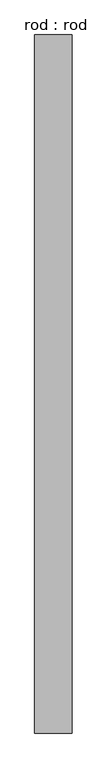
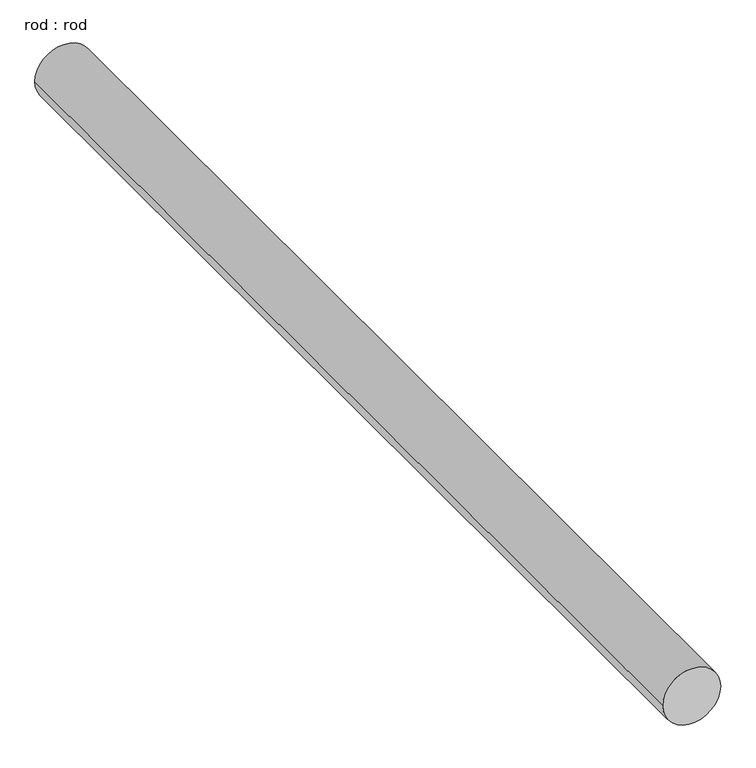
"""IFC4 building model written with IfcOpenShell, lengths in millimetres: proxy geometry, rod : rod."""

import ifcopenshell
import ifcopenshell.guid

model = None  # the IFC model being written
_history = None  # IfcOwnerHistory: only IFC2X3 demands one
_inside = {}  # id of a spatial element -> (the spatial element, [elements in it])
_under = {}  # id of a project, library or spatial element -> (it, [spatial elements below it])
_declared = {}  # id of a project -> (the project, [libraries it declares])
_typed = {}  # id of a type object -> (the type object, [elements of that type])
_made_of = {}  # id of a material, layer set ... -> (it, [elements and type objects made of it])


def new_model(schema):
    """Start an empty IFC model of exactly this schema.

    Asked for "IFC4X3", IfcOpenShell would pick the latest addendum, in which some entities
    have other attributes; the version numbers below select the first issue.
    IFC2X3 requires an IfcOwnerHistory on every rooted entity: one is made here for all.
    """
    global model, _history
    if schema == "IFC4X3":
        model = ifcopenshell.file(schema_version=(4, 3, 0, 0))
    else:
        model = ifcopenshell.file(schema=schema)
    _inside.clear()
    _under.clear()
    _declared.clear()
    _typed.clear()
    _made_of.clear()
    _history = None
    if model.schema == "IFC2X3":
        org = make("IfcOrganization", Name="unknown")
        user = make(
            "IfcPersonAndOrganization",
            ThePerson=make("IfcPerson", FamilyName="unknown"),
            TheOrganization=org,
        )
        app = make(
            "IfcApplication",
            ApplicationDeveloper=org,
            Version="unknown",
            ApplicationFullName="unknown",
            ApplicationIdentifier="unknown",
        )
        _history = make(
            "IfcOwnerHistory",
            OwningUser=user,
            OwningApplication=app,
            ChangeAction="ADDED",
            CreationDate=0,
        )
    return model


def make(cls, **values):
    """One entity of the class cls with the attributes given. An attribute that is None is left unset."""
    return model.create_entity(
        cls, **{name: value for name, value in values.items() if value is not None}
    )


def rooted(cls, **values):
    """An entity with a GlobalId (a new one), such as an element, a storey or a relation."""
    return make(cls, GlobalId=ifcopenshell.guid.new(), OwnerHistory=_history, **values)


def si_unit(unit_type, name, prefix=None):
    """IfcSIUnit, for example si_unit("LENGTHUNIT", "METRE", prefix="MILLI")."""
    return make("IfcSIUnit", UnitType=unit_type, Prefix=prefix, Name=name)


def assignment(units):
    """IfcUnitAssignment: the units of a project."""
    return None if units is None else make("IfcUnitAssignment", Units=units)


def point(xyz):
    """IfcCartesianPoint."""
    return None if xyz is None else make("IfcCartesianPoint", Coordinates=xyz)


def direction(xyz):
    """IfcDirection."""
    return None if xyz is None else make("IfcDirection", DirectionRatios=xyz)


def frame(location, z_axis=None, x_axis=None):
    """IfcAxis2Placement3D, a coordinate frame: its origin and axes. An axis left out is left unset."""
    return make(
        "IfcAxis2Placement3D",
        Location=point(location),
        Axis=direction(z_axis),
        RefDirection=direction(x_axis),
    )


def frame_2d(location, x_axis=None):
    """IfcAxis2Placement2D, a coordinate frame in the plane: its origin and x axis."""
    return make(
        "IfcAxis2Placement2D", Location=point(location), RefDirection=direction(x_axis)
    )


def origin():
    """The frame at (0, 0, 0) with its axes left unset."""
    return frame((0.0, 0.0, 0.0))


def place(relative_to, where):
    """IfcLocalPlacement: puts the frame where relative to a parent placement (None: the world)."""
    return make(
        "IfcLocalPlacement", PlacementRelTo=relative_to, RelativePlacement=where
    )


def context(
    kind, dimensions, precision=None, world=None, true_north=None, identifier=None
):
    """IfcGeometricRepresentationContext, for example the 3D "Model" context."""
    return make(
        "IfcGeometricRepresentationContext",
        ContextIdentifier=identifier,
        ContextType=kind,
        CoordinateSpaceDimension=dimensions,
        Precision=precision,
        WorldCoordinateSystem=world,
        TrueNorth=true_north,
    )


def project(units=None, contexts=None):
    """IfcProject with its units and contexts."""
    return rooted(
        "IfcProject",
        Name="project",
        RepresentationContexts=contexts,
        UnitsInContext=assignment(units),
    )


def spatial(cls, under=None, at=None, **own):
    """A site, building, storey or space (cls), placed at a placement, below another one or the project."""
    s = rooted(cls, ObjectPlacement=at, **own)
    if under is not None:
        _under.setdefault(under.id(), (under, []))[1].append(s)
    return s


def circle_curve(where, radius):
    """IfcCircle in the frame where."""
    return make("IfcCircle", Position=where, Radius=radius)


def trimmed(basis, trim1, trim2, sense, master):
    """IfcTrimmedCurve: the piece of a basis curve between two trims."""
    return make(
        "IfcTrimmedCurve",
        BasisCurve=basis,
        Trim1=trim1,
        Trim2=trim2,
        SenseAgreement=sense,
        MasterRepresentation=master,
    )


def segment(curve, same_sense, transition):
    """IfcCompositeCurveSegment."""
    return make(
        "IfcCompositeCurveSegment",
        Transition=transition,
        SameSense=same_sense,
        ParentCurve=curve,
    )


def composite_curve(segments, self_intersect=None):
    """IfcCompositeCurve: segments joined end to end."""
    return make("IfcCompositeCurve", Segments=segments, SelfIntersect=self_intersect)


def outline(outer, holes=None, kind="AREA"):
    """IfcArbitraryClosedProfileDef: a profile drawn as a closed curve; with holes, ...WithVoids."""
    if holes is None:
        return make("IfcArbitraryClosedProfileDef", ProfileType=kind, OuterCurve=outer)
    return make(
        "IfcArbitraryProfileDefWithVoids",
        ProfileType=kind,
        OuterCurve=outer,
        InnerCurves=holes,
    )


def extrude(swept, where, along, depth):
    """IfcExtrudedAreaSolid: the profile swept, set in the frame where, extruded along a direction by depth."""
    return make(
        "IfcExtrudedAreaSolid",
        SweptArea=swept,
        Position=where,
        ExtrudedDirection=direction(along),
        Depth=depth,
    )


def shape(context_of_items, identifier, shape_type, items):
    """IfcShapeRepresentation: the items that make up one representation, for example the "Body"."""
    return make(
        "IfcShapeRepresentation",
        ContextOfItems=context_of_items,
        RepresentationIdentifier=identifier,
        RepresentationType=shape_type,
        Items=items,
    )


def source(mapping_origin, context_of_items, identifier, shape_type, items):
    """IfcRepresentationMap: a shape defined once, which mapped items show again and again."""
    return make(
        "IfcRepresentationMap",
        MappingOrigin=mapping_origin,
        MappedRepresentation=shape(context_of_items, identifier, shape_type, items),
    )


def transform(
    local_origin,
    x_axis=None,
    y_axis=None,
    z_axis=None,
    scale=None,
    scale2=None,
    scale3=None,
    uniform=True,
):
    """IfcCartesianTransformationOperator3D, or its non-uniform kind. x_axis, y_axis, z_axis: its Axis1, 2, 3."""
    if uniform:
        return make(
            "IfcCartesianTransformationOperator3D",
            Axis1=direction(x_axis),
            Axis2=direction(y_axis),
            LocalOrigin=point(local_origin),
            Scale=scale,
            Axis3=direction(z_axis),
        )
    return make(
        "IfcCartesianTransformationOperator3DnonUniform",
        Axis1=direction(x_axis),
        Axis2=direction(y_axis),
        LocalOrigin=point(local_origin),
        Scale=scale,
        Axis3=direction(z_axis),
        Scale2=scale2,
        Scale3=scale3,
    )


def mapped(mapping_source, mapping_target):
    """IfcMappedItem: shows the shape of a source again, moved by a transform."""
    return make(
        "IfcMappedItem", MappingSource=mapping_source, MappingTarget=mapping_target
    )


def made_of(thing, what):
    """Note that an element or type object is made of a material, layer set ...; save() writes the relation."""
    if what is not None:
        _made_of.setdefault(what.id(), (what, []))[1].append(thing)
    return thing


def element(
    cls,
    number,
    at=None,
    inside=None,
    cuts=None,
    type_object=None,
    material=None,
    context=None,
    identifier="Body",
    shape_type=None,
    held_by="IfcProductDefinitionShape",
    body=None,
    shapes=None,
    **own,
):
    """One element of the class cls, such as IfcWall. Its Tag is "e" and its number.

    at: its placement. inside: the storey or other place that contains it. cuts: it is an
    opening in that element (IfcRelVoidsElement). A single representation is given by context,
    identifier, shape_type and body (its items); several are given by shapes. held_by: the class
    of the entity that holds the representations. save() writes the other relations.
    """
    e = rooted(cls, Tag="e%d" % number, ObjectPlacement=at, **own)
    if body is not None:
        shapes = [shape(context, identifier, shape_type, body)]
    if shapes is not None:
        e.Representation = make(held_by, Representations=shapes)
    if inside is not None:
        _inside.setdefault(inside.id(), (inside, []))[1].append(e)
    if cuts is not None:
        rooted(
            "IfcRelVoidsElement", RelatingBuildingElement=cuts, RelatedOpeningElement=e
        )
    if type_object is not None:
        _typed.setdefault(type_object.id(), (type_object, []))[1].append(e)
    return made_of(e, material)


def aggregate(whole, parts):
    """IfcRelAggregates: a whole, such as a stair, and the parts it consists of."""
    return rooted("IfcRelAggregates", RelatingObject=whole, RelatedObjects=parts)


def save(model, path):
    """Write the relations noted so far, then the file.

    IfcRelAggregates (storeys below a building ...), IfcRelContainedInSpatialStructure (elements
    in a storey), IfcRelDefinesByType, IfcRelAssociatesMaterial and IfcRelDeclares: one each for
    every whole, place, type object, material and project.
    """
    for whole, parts in _under.values():
        aggregate(whole, parts)
    for where, things in _inside.values():
        rooted(
            "IfcRelContainedInSpatialStructure",
            RelatedElements=things,
            RelatingStructure=where,
        )
    for kind, things in _typed.values():
        rooted("IfcRelDefinesByType", RelatedObjects=things, RelatingType=kind)
    for what, things in _made_of.values():
        rooted("IfcRelAssociatesMaterial", RelatedObjects=things, RelatingMaterial=what)
    for by, libraries in _declared.values():
        rooted("IfcRelDeclares", RelatingContext=by, RelatedDefinitions=libraries)
    model.write(path)


def rod_rod_3924ccb1(model_context):
    return source(origin(), model_context, "Body", "SweptSolid", [
        extrude(outline(composite_curve([segment(trimmed(circle_curve(frame_2d((0.0108462, 0.0)), 200.0), [point((0.0108462, 200.0))], [point((0.0108462, -200.0))], False, "CARTESIAN"), True, "CONTINUOUS"), segment(trimmed(circle_curve(frame_2d((0.0108462, 0.0)), 200.0), [point((0.0108462, -200.0))], [point((0.0108462, 200.0))], False, "CARTESIAN"), True, "CONTINUOUS")], self_intersect=False)), frame((0.0, 347.5650675, 0.0), z_axis=(0.0, 1.0, 0.0), x_axis=(0.0, 0.0, 1.0)), (0.0, 0.0, 1.0), 7490.3270957),
    ])


if __name__ == "__main__":
    model = new_model("IFC4")
    model_context = context("Model", 3, world=origin())
    ifc_project = project(units=[si_unit("LENGTHUNIT", "METRE", prefix="MILLI")], contexts=[model_context])
    site = spatial("IfcSite", under=ifc_project)
    building = spatial("IfcBuilding", under=site)
    placement = place(None, origin())
    rod_rod_shape = rod_rod_3924ccb1(model_context)
    element("IfcBuildingElementProxy", 1, Name="rod : rod", ObjectType="rod : rod", at=placement, inside=building, context=model_context, shape_type="MappedRepresentation", body=[
        mapped(rod_rod_shape, transform((0.0, 0.0, 0.0), x_axis=(1.0, 0.0, 0.0), y_axis=(0.0, 1.0, 0.0), z_axis=(0.0, 0.0, 1.0))),
    ])
    save(model, "model.ifc")

# Revit data of these elements
# Type "rod : rod"
#   Default Elevation = 0
